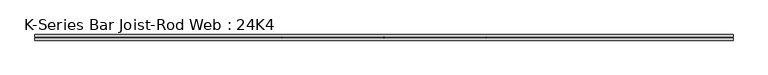
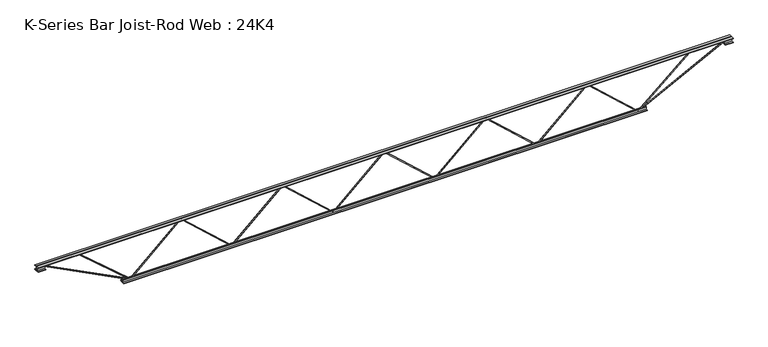
"""IFC4 building model written with IfcOpenShell, lengths in millimetres: beam geometry, K-Series Bar Joist-Rod Web : 24K4."""

from ifc_helpers import new_model, si_unit, frame, origin, place, context, project, spatial, polyline, outline, extrude, source, transform, mapped, element, save


def k_series_bar_joist_rod_web_24k4_98bbd377(model_context):
    return source(origin(), model_context, "Body", "SweptSolid", [
        extrude(outline(polyline([(-293.6875, 662.78125), (-303.2125, 662.78125), (-303.2125, 667.7977947), (293.6875, 1324.2290447), (293.6875, 1326.8959553), (-303.2125, 1983.3272053), (-303.2125, 1988.34375), (-293.6875, 1988.34375), (-293.6875, 1987.0102947), (303.2125, 1330.5790447), (303.2125, 1320.5459553), (-293.6875, 664.1147053), (-293.6875, 662.78125)])), frame((0.0, -4.7625, 0.0), z_axis=(0.0, 1.0, 0.0), x_axis=(0.0, 0.0, 1.0)), (0.0, 0.0, 1.0), 9.525),
        extrude(outline(polyline([(-293.6875, -662.78125), (-303.2125, -662.78125), (-303.2125, -657.7647053), (293.6875, -1.3334553), (293.6875, 1.3334553), (-303.2125, 657.7647053), (-303.2125, 662.78125), (-293.6875, 662.78125), (-293.6875, 661.4477947), (303.2125, 5.0165447), (303.2125, -5.0165447), (-293.6875, -661.4477947), (-293.6875, -662.78125)])), frame((0.0, -4.7625, 0.0), z_axis=(0.0, 1.0, 0.0), x_axis=(0.0, 0.0, 1.0)), (0.0, 0.0, 1.0), 9.525),
        extrude(outline(polyline([(-293.6875, -1988.34375), (-303.2125, -1988.34375), (-303.2125, -1983.3272053), (293.6875, -1326.8959553), (293.6875, -1324.2290447), (-303.2125, -667.7977947), (-303.2125, -662.78125), (-293.6875, -662.78125), (-293.6875, -664.1147053), (303.2125, -1320.5459553), (303.2125, -1330.5790447), (-293.6875, -1987.0102947), (-293.6875, -1988.34375)])), frame((0.0, -4.7625, 0.0), z_axis=(0.0, 1.0, 0.0), x_axis=(0.0, 0.0, 1.0)), (0.0, 0.0, 1.0), 9.525),
        extrude(outline(polyline([(-293.6875, 1988.34375), (-303.2125, 1988.34375), (-303.2125, 1993.3602947), (293.6875, 2649.7915447), (293.6875, 2652.4584553), (-303.2125, 3308.8897053), (-303.2125, 3313.90625), (-293.6875, 3313.90625), (-293.6875, 3312.5727947), (303.2125, 2656.1415447), (303.2125, 2646.1084553), (-293.6875, 1989.6772053), (-293.6875, 1988.34375)])), frame((0.0, -4.7625, 0.0), z_axis=(0.0, 1.0, 0.0), x_axis=(0.0, 0.0, 1.0)), (0.0, 0.0, 1.0), 9.525),
        extrude(outline(polyline([(-293.6875, -3313.90625), (-303.2125, -3313.90625), (-303.2125, -3308.8897053), (293.6875, -2652.4584553), (293.6875, -2649.7915447), (-303.2125, -1993.3602947), (-303.2125, -1988.34375), (-293.6875, -1988.34375), (-293.6875, -1989.6772053), (303.2125, -2646.1084553), (303.2125, -2656.1415447), (-293.6875, -3312.5727947), (-293.6875, -3313.90625)])), frame((0.0, -4.7625, 0.0), z_axis=(0.0, 1.0, 0.0), x_axis=(0.0, 0.0, 1.0)), (0.0, 0.0, 1.0), 9.525),
        extrude(outline(polyline([(4.7625, 304.8), (36.5125, 304.8), (36.5125, 298.45), (11.1125, 298.45), (11.1125, 273.05), (4.7625, 273.05), (4.7625, 304.8)])), frame((-4533.10625, 0.0, 0.0), z_axis=(1.0, 0.0, 0.0), x_axis=(0.0, 1.0, 0.0)), (0.0, 0.0, 1.0), 9066.2125),
        extrude(outline(polyline([(-4.7625, 304.8), (-4.7625, 273.05), (-11.1125, 273.05), (-11.1125, 298.45), (-36.5125, 298.45), (-36.5125, 304.8), (-4.7625, 304.8)])), frame((-4533.10625, 0.0, 0.0), z_axis=(1.0, 0.0, 0.0), x_axis=(0.0, 1.0, 0.0)), (0.0, 0.0, 1.0), 9066.2125),
        extrude(outline(polyline([(-4.7625, 241.3), (-36.5125, 241.3), (-36.5125, 247.65), (-11.1125, 247.65), (-11.1125, 273.05), (-4.7625, 273.05), (-4.7625, 241.3)])), frame((-4533.10625, 0.0, 0.0), z_axis=(1.0, 0.0, 0.0), x_axis=(0.0, 1.0, 0.0)), (0.0, 0.0, 1.0), 101.6),
        extrude(outline(polyline([(36.5125, 241.3), (4.7625, 241.3), (4.7625, 273.05), (11.1125, 273.05), (11.1125, 247.65), (36.5125, 247.65), (36.5125, 241.3)])), frame((-4533.10625, 0.0, 0.0), z_axis=(1.0, 0.0, 0.0), x_axis=(0.0, 1.0, 0.0)), (0.0, 0.0, 1.0), 101.6),
        extrude(outline(polyline([(4.7625, 241.3), (4.7625, 273.05), (11.1125, 273.05), (11.1125, 247.65), (36.5125, 247.65), (36.5125, 241.3), (4.7625, 241.3)])), frame((4431.50625, 0.0, 0.0), z_axis=(1.0, 0.0, 0.0), x_axis=(0.0, 1.0, 0.0)), (0.0, 0.0, 1.0), 101.6),
        extrude(outline(polyline([(-4.7625, 241.3), (-36.5125, 241.3), (-36.5125, 247.65), (-11.1125, 247.65), (-11.1125, 273.05), (-4.7625, 273.05), (-4.7625, 241.3)])), frame((4431.50625, 0.0, 0.0), z_axis=(1.0, 0.0, 0.0), x_axis=(0.0, 1.0, 0.0)), (0.0, 0.0, 1.0), 101.6),
        extrude(outline(polyline([(4.7625, -304.8), (4.7625, -273.05), (11.1125, -273.05), (11.1125, -298.45), (36.5125, -298.45), (36.5125, -304.8), (4.7625, -304.8)])), frame((-3415.50625, 0.0, 0.0), z_axis=(1.0, 0.0, 0.0), x_axis=(0.0, 1.0, 0.0)), (0.0, 0.0, 1.0), 6831.0125),
        extrude(outline(polyline([(-4.7625, -304.8), (-36.5125, -304.8), (-36.5125, -298.45), (-11.1125, -298.45), (-11.1125, -273.05), (-4.7625, -273.05), (-4.7625, -304.8)])), frame((-3415.50625, 0.0, 0.0), z_axis=(1.0, 0.0, 0.0), x_axis=(0.0, 1.0, 0.0)), (0.0, 0.0, 1.0), 6831.0125),
        extrude(outline(polyline([(0.0, -9.525), (0.0, 0.0), (1255.2457966, 0.0), (1255.2457966, -9.525), (0.0, -9.525)])), frame((-4433.6745654, 4.7625, 268.8097388), z_axis=(0.4552893158665214, 0.0, 0.8903435510283628), x_axis=(0.8903435510283628, 0.0, -0.4552893158665214)), (0.0, 0.0, 1.0), 9.525),
        extrude(outline(polyline([(0.0, -9.525), (0.0, 0.0), (875.1521213, 0.0), (875.1521213, -9.525), (0.0, -9.525)])), frame((-3979.7975522, 4.7625, 269.4432034), z_axis=(0.6530293261186303, 0.0, 0.7573326212629743), x_axis=(0.7573326212629743, 0.0, -0.6530293261186303)), (0.0, 0.0, 1.0), 9.525),
        extrude(outline(polyline([(0.0, -9.525), (0.0, 0.0), (1255.2457966, 0.0), (1255.2457966, -9.525), (0.0, -9.525)])), frame((4433.6745654, -4.7625, 268.8097388), z_axis=(-0.4552893158665133, 0.0, 0.890343551028367), x_axis=(-0.890343551028367, 0.0, -0.4552893158665133)), (0.0, 0.0, 1.0), 9.525),
        extrude(outline(polyline([(0.0, -9.525), (0.0, 0.0), (875.1521213, 0.0), (875.1521213, -9.525), (0.0, -9.525)])), frame((3979.7975522, -4.7625, 269.4432034), z_axis=(-0.6530293261186276, 0.0, 0.7573326212629766), x_axis=(-0.7573326212629766, 0.0, -0.6530293261186276)), (0.0, 0.0, 1.0), 9.525),
    ])


if __name__ == "__main__":
    model = new_model("IFC4")
    model_context = context("Model", 3, world=origin())
    ifc_project = project(units=[si_unit("LENGTHUNIT", "METRE", prefix="MILLI")], contexts=[model_context])
    site = spatial("IfcSite", under=ifc_project)
    building = spatial("IfcBuilding", under=site)
    placement = place(None, origin())
    k_series_bar_joist_rod_web_24k4_shape = k_series_bar_joist_rod_web_24k4_98bbd377(model_context)
    element("IfcBeam", 1, ObjectType="K-Series Bar Joist-Rod Web : 24K4", at=placement, inside=building, context=model_context, shape_type="MappedRepresentation", body=[
        mapped(k_series_bar_joist_rod_web_24k4_shape, transform((0.0, 0.0, 0.0), x_axis=(1.0, 0.0, 0.0), y_axis=(0.0, 1.0, 0.0), z_axis=(0.0, 0.0, 1.0))),
    ])
    save(model, "model.ifc")

# Revit data of these elements
# Type "K-Series Bar Joist-Rod Web : 24K4"
#   Assembly Code = "B1010350"
#   Wt = 8.4
#   Web Thickness = 9.525 mm
#   Start Offset [instance default] = 0 mm
#   Start Extension [instance default] = 0 mm
#   Seat Length = 101.6 mm
#   Seat Depth = 63.5 mm
#   PanelArrayLength [instance default] = 4876.8 mm
#   Panel [instance default] = 1219.2 mm
#   End Offset [instance default] = 0 mm
#   End Extension [instance default] = 0 mm
#   End Panel = 1219.2 mm
#   Cord Leg = 31.75 mm
#   Chord Thickness = 6.35 mm
#   Length [instance default] = 7315.2 mm
#   Depth = 609.6 mm
#   PanelArrayNum [instance default] = 4
#   Structural Material = Steel ASTM A500, Grade C, Round
# Element 1 (IfcBeam, "K-Series Bar Joist-Rod Web : 24K4")
#   PanelArrayLength = 6627.812 mm
#   Panel = 1325.562 mm
#   PanelArrayNum = 5
#   Materials on its faces: "Steel ASTM A500, Grade C, Round"
# Materials
#   "Steel ASTM A500, Grade C, Round": class "Metal", colour RGB 202 101 0, transparency 0, Description = "Carbon steel", Cost = 0
